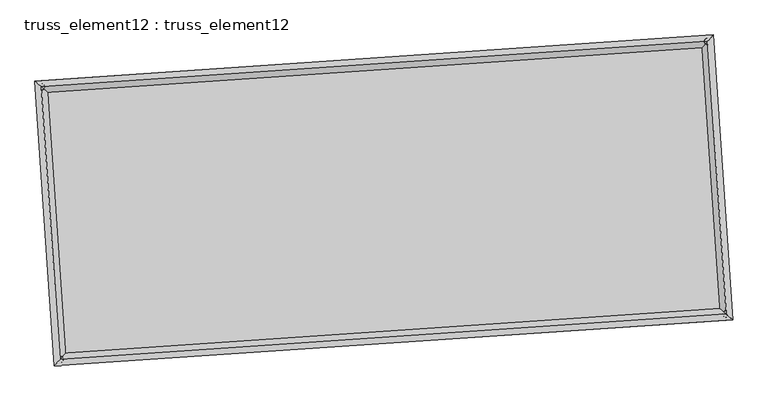
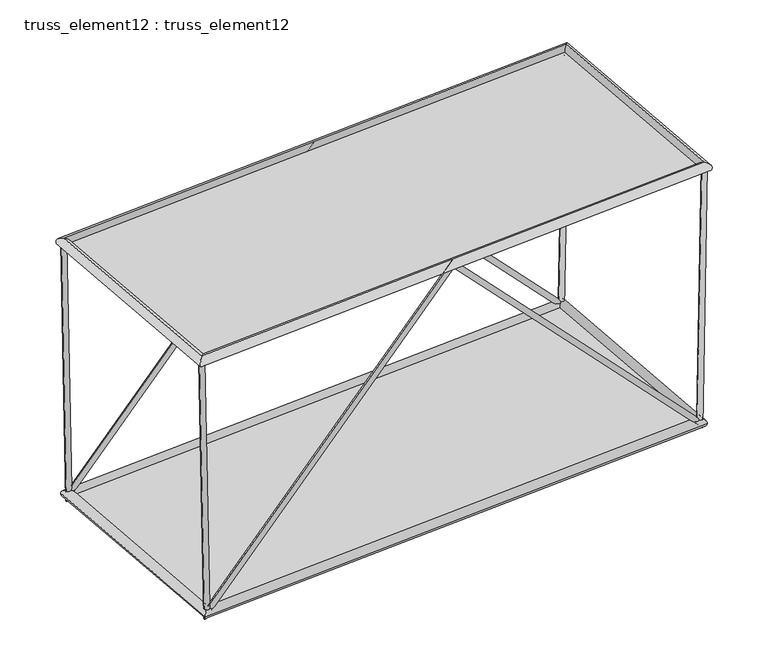
"""IFC4 building model written with IfcOpenShell, lengths in millimetres: plate geometry, truss_element12 : truss_element12."""

import ifcopenshell
import ifcopenshell.guid

model = None  # the IFC model being written
_history = None  # IfcOwnerHistory: only IFC2X3 demands one
_inside = {}  # id of a spatial element -> (the spatial element, [elements in it])
_under = {}  # id of a project, library or spatial element -> (it, [spatial elements below it])
_declared = {}  # id of a project -> (the project, [libraries it declares])
_typed = {}  # id of a type object -> (the type object, [elements of that type])
_made_of = {}  # id of a material, layer set ... -> (it, [elements and type objects made of it])


def new_model(schema):
    """Start an empty IFC model of exactly this schema.

    Asked for "IFC4X3", IfcOpenShell would pick the latest addendum, in which some entities
    have other attributes; the version numbers below select the first issue.
    IFC2X3 requires an IfcOwnerHistory on every rooted entity: one is made here for all.
    """
    global model, _history
    if schema == "IFC4X3":
        model = ifcopenshell.file(schema_version=(4, 3, 0, 0))
    else:
        model = ifcopenshell.file(schema=schema)
    _inside.clear()
    _under.clear()
    _declared.clear()
    _typed.clear()
    _made_of.clear()
    _history = None
    if model.schema == "IFC2X3":
        org = make("IfcOrganization", Name="unknown")
        user = make(
            "IfcPersonAndOrganization",
            ThePerson=make("IfcPerson", FamilyName="unknown"),
            TheOrganization=org,
        )
        app = make(
            "IfcApplication",
            ApplicationDeveloper=org,
            Version="unknown",
            ApplicationFullName="unknown",
            ApplicationIdentifier="unknown",
        )
        _history = make(
            "IfcOwnerHistory",
            OwningUser=user,
            OwningApplication=app,
            ChangeAction="ADDED",
            CreationDate=0,
        )
    return model


def make(cls, **values):
    """One entity of the class cls with the attributes given. An attribute that is None is left unset."""
    return model.create_entity(
        cls, **{name: value for name, value in values.items() if value is not None}
    )


def rooted(cls, **values):
    """An entity with a GlobalId (a new one), such as an element, a storey or a relation."""
    return make(cls, GlobalId=ifcopenshell.guid.new(), OwnerHistory=_history, **values)


def si_unit(unit_type, name, prefix=None):
    """IfcSIUnit, for example si_unit("LENGTHUNIT", "METRE", prefix="MILLI")."""
    return make("IfcSIUnit", UnitType=unit_type, Prefix=prefix, Name=name)


def assignment(units):
    """IfcUnitAssignment: the units of a project."""
    return None if units is None else make("IfcUnitAssignment", Units=units)


def point(xyz):
    """IfcCartesianPoint."""
    return None if xyz is None else make("IfcCartesianPoint", Coordinates=xyz)


def direction(xyz):
    """IfcDirection."""
    return None if xyz is None else make("IfcDirection", DirectionRatios=xyz)


def frame(location, z_axis=None, x_axis=None):
    """IfcAxis2Placement3D, a coordinate frame: its origin and axes. An axis left out is left unset."""
    return make(
        "IfcAxis2Placement3D",
        Location=point(location),
        Axis=direction(z_axis),
        RefDirection=direction(x_axis),
    )


def origin():
    """The frame at (0, 0, 0) with its axes left unset."""
    return frame((0.0, 0.0, 0.0))


def origin_with_axes():
    """The frame at (0, 0, 0) with the z axis (0, 0, 1) and the x axis (1, 0, 0) written out."""
    return frame((0.0, 0.0, 0.0), z_axis=(0.0, 0.0, 1.0), x_axis=(1.0, 0.0, 0.0))


def place(relative_to, where):
    """IfcLocalPlacement: puts the frame where relative to a parent placement (None: the world)."""
    return make(
        "IfcLocalPlacement", PlacementRelTo=relative_to, RelativePlacement=where
    )


def context(
    kind, dimensions, precision=None, world=None, true_north=None, identifier=None
):
    """IfcGeometricRepresentationContext, for example the 3D "Model" context."""
    return make(
        "IfcGeometricRepresentationContext",
        ContextIdentifier=identifier,
        ContextType=kind,
        CoordinateSpaceDimension=dimensions,
        Precision=precision,
        WorldCoordinateSystem=world,
        TrueNorth=true_north,
    )


def project(units=None, contexts=None):
    """IfcProject with its units and contexts."""
    return rooted(
        "IfcProject",
        Name="project",
        RepresentationContexts=contexts,
        UnitsInContext=assignment(units),
    )


def spatial(cls, under=None, at=None, **own):
    """A site, building, storey or space (cls), placed at a placement, below another one or the project."""
    s = rooted(cls, ObjectPlacement=at, **own)
    if under is not None:
        _under.setdefault(under.id(), (under, []))[1].append(s)
    return s


def polyline(points):
    """IfcPolyline through the points."""
    return make("IfcPolyline", Points=[point(p) for p in points])


def circle_curve(where, radius):
    """IfcCircle in the frame where."""
    return make("IfcCircle", Position=where, Radius=radius)


def ellipse_curve(where, semi_axis1, semi_axis2):
    """IfcEllipse in the frame where."""
    return make(
        "IfcEllipse", Position=where, SemiAxis1=semi_axis1, SemiAxis2=semi_axis2
    )


def outline(outer, holes=None, kind="AREA"):
    """IfcArbitraryClosedProfileDef: a profile drawn as a closed curve; with holes, ...WithVoids."""
    if holes is None:
        return make("IfcArbitraryClosedProfileDef", ProfileType=kind, OuterCurve=outer)
    return make(
        "IfcArbitraryProfileDefWithVoids",
        ProfileType=kind,
        OuterCurve=outer,
        InnerCurves=holes,
    )


def extrude(swept, where, along, depth):
    """IfcExtrudedAreaSolid: the profile swept, set in the frame where, extruded along a direction by depth."""
    return make(
        "IfcExtrudedAreaSolid",
        SweptArea=swept,
        Position=where,
        ExtrudedDirection=direction(along),
        Depth=depth,
    )


def shape(context_of_items, identifier, shape_type, items):
    """IfcShapeRepresentation: the items that make up one representation, for example the "Body"."""
    return make(
        "IfcShapeRepresentation",
        ContextOfItems=context_of_items,
        RepresentationIdentifier=identifier,
        RepresentationType=shape_type,
        Items=items,
    )


def source(mapping_origin, context_of_items, identifier, shape_type, items):
    """IfcRepresentationMap: a shape defined once, which mapped items show again and again."""
    return make(
        "IfcRepresentationMap",
        MappingOrigin=mapping_origin,
        MappedRepresentation=shape(context_of_items, identifier, shape_type, items),
    )


def transform(
    local_origin,
    x_axis=None,
    y_axis=None,
    z_axis=None,
    scale=None,
    scale2=None,
    scale3=None,
    uniform=True,
):
    """IfcCartesianTransformationOperator3D, or its non-uniform kind. x_axis, y_axis, z_axis: its Axis1, 2, 3."""
    if uniform:
        return make(
            "IfcCartesianTransformationOperator3D",
            Axis1=direction(x_axis),
            Axis2=direction(y_axis),
            LocalOrigin=point(local_origin),
            Scale=scale,
            Axis3=direction(z_axis),
        )
    return make(
        "IfcCartesianTransformationOperator3DnonUniform",
        Axis1=direction(x_axis),
        Axis2=direction(y_axis),
        LocalOrigin=point(local_origin),
        Scale=scale,
        Axis3=direction(z_axis),
        Scale2=scale2,
        Scale3=scale3,
    )


def mapped(mapping_source, mapping_target):
    """IfcMappedItem: shows the shape of a source again, moved by a transform."""
    return make(
        "IfcMappedItem", MappingSource=mapping_source, MappingTarget=mapping_target
    )


def made_of(thing, what):
    """Note that an element or type object is made of a material, layer set ...; save() writes the relation."""
    if what is not None:
        _made_of.setdefault(what.id(), (what, []))[1].append(thing)
    return thing


def element(
    cls,
    number,
    at=None,
    inside=None,
    cuts=None,
    type_object=None,
    material=None,
    context=None,
    identifier="Body",
    shape_type=None,
    held_by="IfcProductDefinitionShape",
    body=None,
    shapes=None,
    **own,
):
    """One element of the class cls, such as IfcWall. Its Tag is "e" and its number.

    at: its placement. inside: the storey or other place that contains it. cuts: it is an
    opening in that element (IfcRelVoidsElement). A single representation is given by context,
    identifier, shape_type and body (its items); several are given by shapes. held_by: the class
    of the entity that holds the representations. save() writes the other relations.
    """
    e = rooted(cls, Tag="e%d" % number, ObjectPlacement=at, **own)
    if body is not None:
        shapes = [shape(context, identifier, shape_type, body)]
    if shapes is not None:
        e.Representation = make(held_by, Representations=shapes)
    if inside is not None:
        _inside.setdefault(inside.id(), (inside, []))[1].append(e)
    if cuts is not None:
        rooted(
            "IfcRelVoidsElement", RelatingBuildingElement=cuts, RelatedOpeningElement=e
        )
    if type_object is not None:
        _typed.setdefault(type_object.id(), (type_object, []))[1].append(e)
    return made_of(e, material)


def aggregate(whole, parts):
    """IfcRelAggregates: a whole, such as a stair, and the parts it consists of."""
    return rooted("IfcRelAggregates", RelatingObject=whole, RelatedObjects=parts)


def save(model, path):
    """Write the relations noted so far, then the file.

    IfcRelAggregates (storeys below a building ...), IfcRelContainedInSpatialStructure (elements
    in a storey), IfcRelDefinesByType, IfcRelAssociatesMaterial and IfcRelDeclares: one each for
    every whole, place, type object, material and project.
    """
    for whole, parts in _under.values():
        aggregate(whole, parts)
    for where, things in _inside.values():
        rooted(
            "IfcRelContainedInSpatialStructure",
            RelatedElements=things,
            RelatingStructure=where,
        )
    for kind, things in _typed.values():
        rooted("IfcRelDefinesByType", RelatedObjects=things, RelatingType=kind)
    for what, things in _made_of.values():
        rooted("IfcRelAssociatesMaterial", RelatedObjects=things, RelatingMaterial=what)
    for by, libraries in _declared.values():
        rooted("IfcRelDeclares", RelatingContext=by, RelatedDefinitions=libraries)
    model.write(path)


def plane_surface(at):
    """IfcPlane: the flat surface through the origin of the frame at, square to its z axis."""
    return make("IfcPlane", Position=at)


def cylinder_surface(at, radius):
    """IfcCylindricalSurface: all points at the distance radius from the z axis of the frame at."""
    return make("IfcCylindricalSurface", Position=at, Radius=radius)


def advanced_brep(points, edges, surfaces, faces):
    """IfcAdvancedBrep: a solid bounded by faces that lie on surfaces and meet in shared edges.

    An edge is (start, end): straight between two places in points (the first is 0);
    or (start, end, curve); or (start, end, curve, False) where it runs against its curve.
    A face is (place in surfaces, loops), or (place, loops, False) where it looks against
    its surface's normal. A loop lists edges by number (the first is 1), with a minus sign
    where the edge is run from its end to its start. The first loop is the outer one.
    """
    corners = [point(p) for p in points]
    vertices = [make("IfcVertexPoint", VertexGeometry=c) for c in corners]
    made = []
    for start, end, *more in edges:
        made.append(
            make(
                "IfcEdgeCurve",
                EdgeStart=vertices[start],
                EdgeEnd=vertices[end],
                EdgeGeometry=more[0] if more else make("IfcPolyline", Points=[corners[start], corners[end]]),
                SameSense=more[1] if len(more) > 1 else True,
            )
        )
    hull = []
    for where, loops, *sense in faces:
        bounds = []
        for j, loop in enumerate(loops):
            ring = [make("IfcOrientedEdge", EdgeElement=made[abs(k) - 1], Orientation=k > 0) for k in loop]
            bounds.append(
                make(
                    "IfcFaceOuterBound" if j == 0 else "IfcFaceBound",
                    Bound=make("IfcEdgeLoop", EdgeList=ring),
                    Orientation=True,
                )
            )
        hull.append(make("IfcAdvancedFace", Bounds=bounds, FaceSurface=surfaces[where], SameSense=sense[0] if sense else True))
    return make("IfcAdvancedBrep", Outer=make("IfcClosedShell", CfsFaces=hull))


def truss_element12_truss_element12_4f4fbcf4(model_context):
    return source(origin(), model_context, "Body", "SolidModel", [
        advanced_brep(
        [(-3760.412313, 2269.7141982, 5000.0391427), (-3859.4974462, 2256.3541767, 4998.1296386), (-3667.2581462, 2276.0660267, 121.7809681), (-3761.7287366, 2263.0206534, -121.7809681), (1063.0131777, 2598.6052469, 5071.2149086), (1063.4719257, 2592.0327442, 4926.9805708), (5794.6632736, 2921.2384802, 121.7906375), (5890.0977034, 2921.1420083, -121.7906375), (5886.4489476, 2927.4969964, 5000.0518193), (5986.4310183, 2927.7106108, 4998.1703582)],
        [
            (0, 1, circle_curve(frame((-3809.9548796, 2263.0341875, 4999.0843906), z_axis=(-0.01909228763423125, -0.001301830517198407, 0.9998168781282883), x_axis=(-0.13360060813890293, 0.9910344534146752, -0.0012608132261237302)), 50.0)),
            (1, 0, circle_curve(frame((-3809.9548796, 2263.0341875, 4999.0843906), z_axis=(-0.01909228763423125, -0.001301830517198407, 0.9998168781282883), x_axis=(-0.13360060813890293, 0.9910344534146752, -0.0012608132261237302)), 50.0)),
            (0, 2),
            (2, 3, ellipse_curve(frame((-3714.4934414, 2269.54334, 0.0), z_axis=(-0.9293023610631932, -0.06336559539190412, 0.36384326713985493), x_axis=(0.36300038639906895, 0.02475161645489898, 0.9314601853847518)), 131.026691, 50.0)),
            (3, 1),
            (3, 2, ellipse_curve(frame((-3714.4934414, 2269.54334, 0.0), z_axis=(-0.9293023610631932, -0.06336559539190412, 0.36384326713985493), x_axis=(0.36300038639906895, 0.02475161645489898, 0.9314601853847518)), 131.026691, 50.0)),
            (2, 4),
            (4, 5, ellipse_curve(frame((1063.2425517, 2595.3189955, 4999.0977397), z_axis=(-0.9976833933961032, -0.0680282380460461, -7.328019523158009e-05), x_axis=(7.311043404377707e-05, 4.985122578964847e-06, -0.9999999973150066)), 72.2742041, 50.0)),
            (5, 3),
            (5, 4, ellipse_curve(frame((1063.2425517, 2595.3189955, 4999.0977397), z_axis=(-0.9976833933961032, -0.0680282380460461, -7.328019523158009e-05), x_axis=(7.311043404377707e-05, 4.985122578964847e-06, -0.9999999973150066)), 72.2742041, 50.0)),
            (4, 6),
            (6, 7, ellipse_curve(frame((5842.3804885, 2921.1902443, 0.0), z_axis=(-0.9292247210951414, -0.06336030141762011, -0.36404242872215437), x_axis=(-0.36319908660286526, -0.02476516506646599, 0.9313823651380109)), 131.0480431, 50.0)),
            (7, 5),
            (7, 6, ellipse_curve(frame((5842.3804885, 2921.1902443, 0.0), z_axis=(-0.9292247210951414, -0.06336030141762011, -0.36404242872215437), x_axis=(-0.36319908660286526, -0.02476516506646599, 0.9313823651380109)), 131.0480431, 50.0)),
            (8, 9, circle_curve(frame((5936.4399829, 2927.6038036, 4999.1110888), z_axis=(0.018811898886609116, 0.0012827118743552863, 0.9998222177519999), x_axis=(-0.002159898325700627, 0.9999968957639224, -0.001242296961952952)), 50.0)),
            (9, 8, circle_curve(frame((5936.4399829, 2927.6038036, 4999.1110888), z_axis=(0.018811898886609116, 0.0012827118743552863, 0.9998222177519999), x_axis=(-0.002159898325700627, 0.9999968957639224, -0.001242296961952952)), 50.0)),
            (6, 8),
            (9, 7),
        ],
        [
            plane_surface(frame((-3809.9548796, 2313.0341451, 4999.149494), z_axis=(-0.019092287634232964, -0.0013018305172036876, 0.9998168781282883), x_axis=(0.9998177256644792, -2.4859453925607497e-05, 0.01909227144987823))),
            cylinder_surface(frame((-3809.9548796, 2263.0341875, 4999.0843906), z_axis=(-0.019092287634231247, -0.0013018305171984068, 0.9998168781282881), x_axis=(-0.13360060813890293, 0.9910344534146752, -0.0012608132261237302)), 50.0),
            cylinder_surface(frame((-3714.4934414, 2269.54334, 0.0), z_axis=(-0.690154320065974, -0.047058999563115655, -0.7221305041710897), x_axis=(-0.020413190140967315, 0.9987522731822975, -0.04557629297630685)), 50.0),
            cylinder_surface(frame((1063.2425517, 2595.3189955, 4999.0977397), z_axis=(-0.6902599032026433, -0.04706619887584647, 0.7220291122621422), x_axis=(-0.11534100259403575, 0.9922795065055209, -0.04558326545743215)), 50.0),
            plane_surface(frame((5936.4399829, 2877.6038448, 4999.1752357), z_axis=(0.018811898886608048, 0.0012827118743585436, 0.9998222177519999), x_axis=(0.9998230405728206, -2.41345169111895e-05, -0.018811883405046356))),
            cylinder_surface(frame((5842.3804885, 2921.1902443, 0.0), z_axis=(-0.018811898886609116, -0.0012827118743552863, -0.9998222177519999), x_axis=(-0.002159898325700627, 0.9999968957639224, -0.001242296961952952)), 50.0),
        ],
        [
            (0, [[1, 2]]),
            (1, [[-1, 3, 4, 5]]),
            (1, [[-2, -5, 6, -3]]),
            (2, [[-4, 7, 8, 9]]),
            (2, [[-6, -9, 10, -7]]),
            (3, [[-8, 11, 12, 13]]),
            (3, [[-10, -13, 14, -11]]),
            (4, [[15, 16]]),
            (5, [[-12, 17, -16, 18]]),
            (5, [[-14, -18, -15, -17]]),
        ],
    ),
        advanced_brep(
        [(-3488.2993601, -1721.0193861, 5000.0391427), (-3587.3844933, -1734.3794076, 4998.1296386), (-3395.1451933, -1714.6675576, 121.7809681), (-3489.6157837, -1727.7129309, -121.7809681), (1335.1261306, -1392.1283374, 5071.2149086), (1335.5848786, -1398.7008401, 4926.9805708), (6066.7762265, -1069.4951041, 121.7906375), (6162.2106563, -1069.591576, -121.7906375), (6158.5619005, -1063.2365879, 5000.0518193), (6258.5439712, -1063.0229735, 4998.1703582)],
        [
            (0, 1, circle_curve(frame((-3537.8419267, -1727.6993968, 4999.0843906), z_axis=(-0.019092287634231597, -0.0013018305171984207, 0.9998168781282882), x_axis=(-0.13360060813890337, 0.9910344534146753, -0.001260813226123772)), 50.0)),
            (1, 0, circle_curve(frame((-3537.8419267, -1727.6993968, 4999.0843906), z_axis=(-0.019092287634231597, -0.0013018305171984207, 0.9998168781282882), x_axis=(-0.13360060813890337, 0.9910344534146753, -0.001260813226123772)), 50.0)),
            (0, 2),
            (2, 3, ellipse_curve(frame((-3442.3804885, -1721.1902443, 0.0), z_axis=(-0.9293023610631933, -0.06336559539190433, 0.36384326713985427), x_axis=(0.3630003863990683, 0.02475161645489903, 0.9314601853847522)), 131.026691, 50.0)),
            (3, 1),
            (3, 2, ellipse_curve(frame((-3442.3804885, -1721.1902443, 0.0), z_axis=(-0.9293023610631933, -0.06336559539190433, 0.36384326713985427), x_axis=(0.3630003863990683, 0.02475161645489903, 0.9314601853847522)), 131.026691, 50.0)),
            (2, 4),
            (4, 5, ellipse_curve(frame((1335.3555046, -1395.4145888, 4999.0977397), z_axis=(-0.9976833933961031, -0.06802823804604609, -7.328019523141967e-05), x_axis=(7.311043404362326e-05, 4.985122578705385e-06, -0.9999999973150066)), 72.2742041, 50.0)),
            (5, 3),
            (5, 4, ellipse_curve(frame((1335.3555046, -1395.4145888, 4999.0977397), z_axis=(-0.9976833933961031, -0.06802823804604609, -7.328019523141967e-05), x_axis=(7.311043404362326e-05, 4.985122578705385e-06, -0.9999999973150066)), 72.2742041, 50.0)),
            (4, 6),
            (6, 7, ellipse_curve(frame((6114.4934414, -1069.54334, 0.0), z_axis=(-0.9292247210951415, -0.06336030141762007, -0.36404242872215387), x_axis=(-0.3631990866028648, -0.024765165066465773, 0.9313823651380111)), 131.0480431, 50.0)),
            (7, 5),
            (7, 6, ellipse_curve(frame((6114.4934414, -1069.54334, 0.0), z_axis=(-0.9292247210951415, -0.06336030141762007, -0.36404242872215387), x_axis=(-0.3631990866028648, -0.024765165066465773, 0.9313823651380111)), 131.0480431, 50.0)),
            (8, 9, circle_curve(frame((6208.5529358, -1063.1297807, 4999.1110888), z_axis=(0.018811898886609498, 0.0012827118743554589, 0.9998222177519999), x_axis=(-0.002159898325700537, 0.9999968957639224, -0.0012422969619531254)), 50.0)),
            (9, 8, circle_curve(frame((6208.5529358, -1063.1297807, 4999.1110888), z_axis=(0.018811898886609498, 0.0012827118743554589, 0.9998222177519999), x_axis=(-0.002159898325700537, 0.9999968957639224, -0.0012422969619531254)), 50.0)),
            (6, 8),
            (9, 7),
        ],
        [
            plane_surface(frame((-3537.8419267, -1677.6994392, 4999.149494), z_axis=(-0.019092287634232964, -0.001301830517203691, 0.9998168781282883), x_axis=(0.9998177256644792, -2.4859453925607497e-05, 0.01909227144987823))),
            cylinder_surface(frame((-3537.8419267, -1727.6993968, 4999.0843906), z_axis=(-0.0190922876342316, -0.001301830517198421, 0.9998168781282885), x_axis=(-0.13360060813890337, 0.9910344534146753, -0.001260813226123772)), 50.0),
            cylinder_surface(frame((-3442.3804885, -1721.1902443, 0.0), z_axis=(-0.6901543200659737, -0.047058999563115794, -0.7221305041710899), x_axis=(-0.02041319014096742, 0.9987522731822974, -0.04557629297630694)), 50.0),
            cylinder_surface(frame((1335.3555046, -1395.4145888, 4999.0977397), z_axis=(-0.6902599032026426, -0.04706619887584624, 0.7220291122621428), x_axis=(-0.11534100259403567, 0.9922795065055209, -0.045583265457432236)), 50.0),
            plane_surface(frame((6208.5529358, -1113.1297395, 4999.1752357), z_axis=(0.018811898886608048, 0.0012827118743585436, 0.9998222177519999), x_axis=(0.9998230405728206, -2.41345169111895e-05, -0.018811883405046356))),
            cylinder_surface(frame((6114.4934414, -1069.54334, 0.0), z_axis=(-0.018811898886609498, -0.0012827118743554589, -0.9998222177519999), x_axis=(-0.002159898325700537, 0.9999968957639224, -0.0012422969619531254)), 50.0),
        ],
        [
            (0, [[1, 2]]),
            (1, [[-1, 3, 4, 5]]),
            (1, [[-2, -5, 6, -3]]),
            (2, [[-4, 7, 8, 9]]),
            (2, [[-6, -9, 10, -7]]),
            (3, [[-8, 11, 12, 13]]),
            (3, [[-10, -13, 14, -11]]),
            (4, [[15, 16]]),
            (5, [[-12, 17, -16, 18]]),
            (5, [[-14, -18, -15, -17]]),
        ],
    ),
        advanced_brep(
        [(-3537.8349665, -1727.6916826, 4909.084391), (-3537.8488868, -1727.7071111, 5089.0843903), (-3809.9628225, 2263.0408855, 5089.0843903), (-3809.9469367, 2263.0274894, 4909.084391), (5936.4464523, 2927.6114844, 5089.1110885), (5936.4335136, 2927.5961229, 4909.111089), (6208.5603879, -1063.1365122, 5089.1110885), (6208.5454838, -1063.1230492, 4909.111089)],
        [
            (0, 1, ellipse_curve(frame((-3537.8419267, -1727.6993968, 4999.0843906), z_axis=(-0.7535719234028239, 0.6573654662782598, -1.9324773013398396e-06), x_axis=(-0.6573654662754455, -0.753571923405279, -1.9324773013398426e-06)), 127.2792206, 90.0)),
            (1, 2),
            (2, 3, ellipse_curve(frame((-3809.9548796, 2263.0341875, 4999.0843906), z_axis=(-0.6573654662754456, -0.753571923405279, -1.9324773013398405e-06), x_axis=(0.753571923402824, -0.6573654662782596, 1.932477301339838e-06)), 127.2792206, 90.0)),
            (3, 0),
            (1, 0, ellipse_curve(frame((-3537.8419267, -1727.6993968, 4999.0843906), z_axis=(-0.7535719234028239, 0.6573654662782598, -1.9324773013398396e-06), x_axis=(-0.6573654662754455, -0.753571923405279, -1.9324773013398426e-06)), 127.2792206, 90.0)),
            (3, 2, ellipse_curve(frame((-3809.9548796, 2263.0341875, 4999.0843906), z_axis=(-0.6573654662754456, -0.753571923405279, -1.9324773013398405e-06), x_axis=(0.753571923402824, -0.6573654662782596, 1.932477301339838e-06)), 127.2792206, 90.0)),
            (2, 4),
            (4, 5, ellipse_curve(frame((5936.4399829, 2927.6038036, 4999.1110888), z_axis=(-0.7535719234028233, 0.6573654662782605, -1.9324773013398405e-06), x_axis=(-0.6573654662754463, -0.753571923405278, -1.9324773013398375e-06)), 127.2792206, 90.0)),
            (5, 3),
            (5, 4, ellipse_curve(frame((5936.4399829, 2927.6038036, 4999.1110888), z_axis=(-0.7535719234028233, 0.6573654662782605, -1.9324773013398405e-06), x_axis=(-0.6573654662754463, -0.753571923405278, -1.9324773013398375e-06)), 127.2792206, 90.0)),
            (4, 6),
            (6, 7, ellipse_curve(frame((6208.5529358, -1063.1297807, 4999.1110888), z_axis=(0.6573654662754466, 0.753571923405278, 1.9324773013398396e-06), x_axis=(-0.7535719234028231, 0.6573654662782609, -1.9324773013398426e-06)), 127.2792206, 90.0)),
            (7, 5),
            (7, 6, ellipse_curve(frame((6208.5529358, -1063.1297807, 4999.1110888), z_axis=(0.6573654662754466, 0.753571923405278, 1.9324773013398396e-06), x_axis=(-0.7535719234028231, 0.6573654662782609, -1.9324773013398426e-06)), 127.2792206, 90.0)),
            (6, 1),
            (0, 7),
        ],
        [
            cylinder_surface(frame((-3537.8419267, -1727.6993968, 4999.0843906), z_axis=(0.06802823822870284, -0.9976833960748765, 0.0), x_axis=(-0.9976833926394355, -0.06802823799445316, -8.298696276640426e-05)), 90.0),
            cylinder_surface(frame((-3809.9548796, 2263.0341875, 4999.0843906), z_axis=(-0.9976833960711509, -0.06802823822844752, -2.732935608532959e-06), x_axis=(-0.06802823779080554, 0.997683392876903, -8.025402716667233e-05)), 90.0),
            cylinder_surface(frame((5936.4399829, 2927.6038036, 4999.1110888), z_axis=(-0.06802823822870042, 0.9976833960748767, 0.0), x_axis=(0.9976833930770777, 0.0680282380242919, -7.752109156694041e-05)), 90.0),
            cylinder_surface(frame((6208.5529358, -1063.1297807, 4999.1110888), z_axis=(0.9976833960711509, 0.0680282382284473, 2.732935608532962e-06), x_axis=(0.0680282382284473, -0.997683392847062, -8.025402716667235e-05)), 90.0),
        ],
        [
            (0, [[1, 2, 3, 4]]),
            (0, [[5, -4, 6, -2]]),
            (1, [[-3, 7, 8, 9]]),
            (1, [[-6, -9, 10, -7]]),
            (2, [[-8, 11, 12, 13]]),
            (2, [[-10, -13, 14, -11]]),
            (3, [[-12, 15, -1, 16]]),
            (3, [[-14, -16, -5, -15]]),
        ],
    ),
        advanced_brep(
        [(-3358.7115243, -1625.2761972, 0.0), (-3526.0494527, -1817.1042913, 0.0), (-3810.4074885, 2353.2123043, 0.0), (-3618.5793943, 2185.8743758, 0.0), (5926.0494527, 3017.1042913, 0.0), (5758.7115243, 2825.2761972, 0.0), (6210.4074885, -1153.2123043, 0.0), (6018.5793943, -985.8743758, 0.0)],
        [
            (0, 1, ellipse_curve(frame((-3442.3804885, -1721.1902443, 0.0), z_axis=(-0.7535719234054584, 0.6573654662780802, 0.0), x_axis=(-0.6573654662780803, -0.7535719234054584, 0.0)), 127.2792206, 90.0)),
            (1, 2),
            (2, 3, ellipse_curve(frame((-3714.4934414, 2269.54334, 0.0), z_axis=(-0.65736546627808, -0.7535719234054585, 0.0), x_axis=(0.7535719234054585, -0.6573654662780801, 0.0)), 127.2792206, 90.0)),
            (3, 0),
            (1, 0, ellipse_curve(frame((-3442.3804885, -1721.1902443, 0.0), z_axis=(-0.7535719234054584, 0.6573654662780802, 0.0), x_axis=(-0.6573654662780803, -0.7535719234054584, 0.0)), 127.2792206, 90.0)),
            (3, 2, ellipse_curve(frame((-3714.4934414, 2269.54334, 0.0), z_axis=(-0.65736546627808, -0.7535719234054585, 0.0), x_axis=(0.7535719234054585, -0.6573654662780801, 0.0)), 127.2792206, 90.0)),
            (2, 4),
            (4, 5, ellipse_curve(frame((5842.3804885, 2921.1902443, 0.0), z_axis=(-0.7535719234054579, 0.657365466278081, 0.0), x_axis=(-0.657365466278081, -0.7535719234054579, 0.0)), 127.2792206, 90.0)),
            (5, 3),
            (5, 4, ellipse_curve(frame((5842.3804885, 2921.1902443, 0.0), z_axis=(-0.7535719234054579, 0.657365466278081, 0.0), x_axis=(-0.657365466278081, -0.7535719234054579, 0.0)), 127.2792206, 90.0)),
            (4, 6),
            (6, 7, ellipse_curve(frame((6114.4934414, -1069.54334, 0.0), z_axis=(0.6573654662780812, 0.7535719234054576, 0.0), x_axis=(-0.7535719234054576, 0.6573654662780812, 0.0)), 127.2792206, 90.0)),
            (7, 5),
            (7, 6, ellipse_curve(frame((6114.4934414, -1069.54334, 0.0), z_axis=(0.6573654662780812, 0.7535719234054576, 0.0), x_axis=(-0.7535719234054576, 0.6573654662780812, 0.0)), 127.2792206, 90.0)),
            (6, 1),
            (0, 7),
        ],
        [
            cylinder_surface(frame((-3442.3804885, -1721.1902443, 0.0), z_axis=(0.06802823822870306, -0.9976833960748764, 0.0), x_axis=(-0.9976833960748764, -0.06802823822870306, 0.0)), 90.0),
            cylinder_surface(frame((-3714.4934414, 2269.54334, 0.0), z_axis=(-0.9976833960748767, -0.06802823822870151, 0.0), x_axis=(-0.06802823822870151, 0.9976833960748767, 0.0)), 90.0),
            cylinder_surface(frame((5842.3804885, 2921.1902443, 0.0), z_axis=(-0.06802823822870056, 0.9976833960748768, 0.0), x_axis=(0.9976833960748768, 0.06802823822870056, 0.0)), 90.0),
            cylinder_surface(frame((6114.4934414, -1069.54334, 0.0), z_axis=(0.9976833960748768, 0.0680282382287009, 0.0), x_axis=(0.0680282382287009, -0.9976833960748768, 0.0)), 90.0),
        ],
        [
            (0, [[1, 2, 3, 4]]),
            (0, [[5, -4, 6, -2]]),
            (1, [[-3, 7, 8, 9]]),
            (1, [[-6, -9, 10, -7]]),
            (2, [[-8, 11, 12, 13]]),
            (2, [[-10, -13, 14, -11]]),
            (3, [[-12, 15, -1, 16]]),
            (3, [[-14, -16, -5, -15]]),
        ],
    ),
        extrude(outline(polyline([(-3442.3804885, -1721.1902443), (-3714.4934414, 2269.54334), (5842.3804885, 2921.1902443), (6114.4934414, -1069.54334), (-3442.3804885, -1721.1902443)])), origin_with_axes(), (0.0, 0.0, 1.0), 20.0),
        extrude(outline(polyline([(-2000.0, 4884.5129131), (2000.0, 4884.512913), (2000.0, -4884.5129131), (-2000.0, -4884.512913), (-2000.0, 4884.5129131)])), frame((1199.2990281, 599.9522034, 4999.0977397), z_axis=(-2.726604479175121e-06, -1.8591679464098493e-07, 0.9999999999962655), x_axis=(-0.0680282382287028, 0.9976833960748764, 0.0)), (0.0, 0.0, 1.0), 20.0),
    ])


if __name__ == "__main__":
    model = new_model("IFC4")
    model_context = context("Model", 3, world=origin())
    ifc_project = project(units=[si_unit("LENGTHUNIT", "METRE", prefix="MILLI")], contexts=[model_context])
    site = spatial("IfcSite", under=ifc_project)
    building = spatial("IfcBuilding", under=site)
    placement = place(None, origin())
    truss_element12_truss_element12_shape = truss_element12_truss_element12_4f4fbcf4(model_context)
    element("IfcPlate", 1, ObjectType="truss_element12 : truss_element12", at=placement, inside=building, context=model_context, shape_type="MappedRepresentation", body=[
        mapped(truss_element12_truss_element12_shape, transform((0.0, 0.0, 0.0), x_axis=(1.0, 0.0, 0.0), y_axis=(0.0, 1.0, 0.0), z_axis=(0.0, 0.0, 1.0))),
    ])
    save(model, "model.ifc")

# Revit data of these elements
# Project information
#   Project Issue Date = "Issue Date"
#   Project Status = "Project Status"
#   Client Name = "Owner"
#   Project Address = "Enter address here"
#   Project Name = "Project Name"
#   Project Number = "Project Number"
# Type "truss_element12 : truss_element12"
#   steellbar1 = 90 mm
#   steelbar2 = 50 mm
#   offset1 = 5000 mm
#   M = Default Roof
# Element 1 (IfcPlate, "truss_element12 : truss_element12")
#   Materials on its faces: "Default Roof"
# Materials
#   "Default Roof": class "Miscellaneous", colour RGB 0 127 0, transparency 0, Comments = "Rendering appearance not upgraded Rendering appearance not upgraded ", Cost = 0
